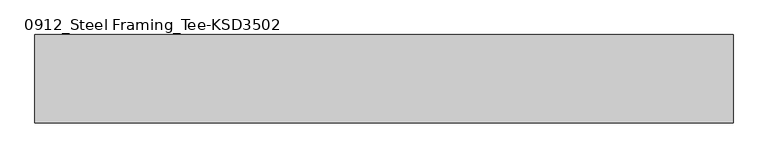
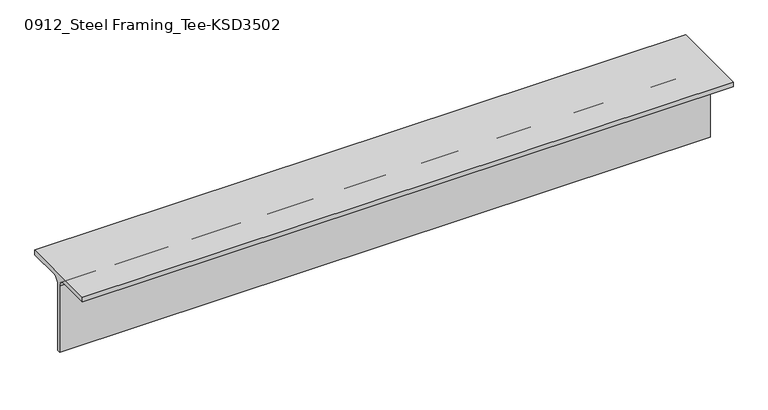
"""IFC4 building model written with IfcOpenShell, lengths in millimetres: member geometry, 0912_Steel Framing_Tee-KSD3502 : H_SB_ASB_CT-150x150x6.5x9."""

import ifcopenshell
import ifcopenshell.guid

model = None  # the IFC model being written
_history = None  # IfcOwnerHistory: only IFC2X3 demands one
_inside = {}  # id of a spatial element -> (the spatial element, [elements in it])
_under = {}  # id of a project, library or spatial element -> (it, [spatial elements below it])
_declared = {}  # id of a project -> (the project, [libraries it declares])
_typed = {}  # id of a type object -> (the type object, [elements of that type])
_made_of = {}  # id of a material, layer set ... -> (it, [elements and type objects made of it])


def new_model(schema):
    """Start an empty IFC model of exactly this schema.

    Asked for "IFC4X3", IfcOpenShell would pick the latest addendum, in which some entities
    have other attributes; the version numbers below select the first issue.
    IFC2X3 requires an IfcOwnerHistory on every rooted entity: one is made here for all.
    """
    global model, _history
    if schema == "IFC4X3":
        model = ifcopenshell.file(schema_version=(4, 3, 0, 0))
    else:
        model = ifcopenshell.file(schema=schema)
    _inside.clear()
    _under.clear()
    _declared.clear()
    _typed.clear()
    _made_of.clear()
    _history = None
    if model.schema == "IFC2X3":
        org = make("IfcOrganization", Name="unknown")
        user = make(
            "IfcPersonAndOrganization",
            ThePerson=make("IfcPerson", FamilyName="unknown"),
            TheOrganization=org,
        )
        app = make(
            "IfcApplication",
            ApplicationDeveloper=org,
            Version="unknown",
            ApplicationFullName="unknown",
            ApplicationIdentifier="unknown",
        )
        _history = make(
            "IfcOwnerHistory",
            OwningUser=user,
            OwningApplication=app,
            ChangeAction="ADDED",
            CreationDate=0,
        )
    return model


def make(cls, **values):
    """One entity of the class cls with the attributes given. An attribute that is None is left unset."""
    return model.create_entity(
        cls, **{name: value for name, value in values.items() if value is not None}
    )


def rooted(cls, **values):
    """An entity with a GlobalId (a new one), such as an element, a storey or a relation."""
    return make(cls, GlobalId=ifcopenshell.guid.new(), OwnerHistory=_history, **values)


def si_unit(unit_type, name, prefix=None):
    """IfcSIUnit, for example si_unit("LENGTHUNIT", "METRE", prefix="MILLI")."""
    return make("IfcSIUnit", UnitType=unit_type, Prefix=prefix, Name=name)


def assignment(units):
    """IfcUnitAssignment: the units of a project."""
    return None if units is None else make("IfcUnitAssignment", Units=units)


def point(xyz):
    """IfcCartesianPoint."""
    return None if xyz is None else make("IfcCartesianPoint", Coordinates=xyz)


def direction(xyz):
    """IfcDirection."""
    return None if xyz is None else make("IfcDirection", DirectionRatios=xyz)


def frame(location, z_axis=None, x_axis=None):
    """IfcAxis2Placement3D, a coordinate frame: its origin and axes. An axis left out is left unset."""
    return make(
        "IfcAxis2Placement3D",
        Location=point(location),
        Axis=direction(z_axis),
        RefDirection=direction(x_axis),
    )


def frame_2d(location, x_axis=None):
    """IfcAxis2Placement2D, a coordinate frame in the plane: its origin and x axis."""
    return make(
        "IfcAxis2Placement2D", Location=point(location), RefDirection=direction(x_axis)
    )


def origin():
    """The frame at (0, 0, 0) with its axes left unset."""
    return frame((0.0, 0.0, 0.0))


def place(relative_to, where):
    """IfcLocalPlacement: puts the frame where relative to a parent placement (None: the world)."""
    return make(
        "IfcLocalPlacement", PlacementRelTo=relative_to, RelativePlacement=where
    )


def context(
    kind, dimensions, precision=None, world=None, true_north=None, identifier=None
):
    """IfcGeometricRepresentationContext, for example the 3D "Model" context."""
    return make(
        "IfcGeometricRepresentationContext",
        ContextIdentifier=identifier,
        ContextType=kind,
        CoordinateSpaceDimension=dimensions,
        Precision=precision,
        WorldCoordinateSystem=world,
        TrueNorth=true_north,
    )


def project(units=None, contexts=None):
    """IfcProject with its units and contexts."""
    return rooted(
        "IfcProject",
        Name="project",
        RepresentationContexts=contexts,
        UnitsInContext=assignment(units),
    )


def spatial(cls, under=None, at=None, **own):
    """A site, building, storey or space (cls), placed at a placement, below another one or the project."""
    s = rooted(cls, ObjectPlacement=at, **own)
    if under is not None:
        _under.setdefault(under.id(), (under, []))[1].append(s)
    return s


def polyline(points):
    """IfcPolyline through the points."""
    return make("IfcPolyline", Points=[point(p) for p in points])


def circle_curve(where, radius):
    """IfcCircle in the frame where."""
    return make("IfcCircle", Position=where, Radius=radius)


def trimmed(basis, trim1, trim2, sense, master):
    """IfcTrimmedCurve: the piece of a basis curve between two trims."""
    return make(
        "IfcTrimmedCurve",
        BasisCurve=basis,
        Trim1=trim1,
        Trim2=trim2,
        SenseAgreement=sense,
        MasterRepresentation=master,
    )


def segment(curve, same_sense, transition):
    """IfcCompositeCurveSegment."""
    return make(
        "IfcCompositeCurveSegment",
        Transition=transition,
        SameSense=same_sense,
        ParentCurve=curve,
    )


def composite_curve(segments, self_intersect=None):
    """IfcCompositeCurve: segments joined end to end."""
    return make("IfcCompositeCurve", Segments=segments, SelfIntersect=self_intersect)


def outline(outer, holes=None, kind="AREA"):
    """IfcArbitraryClosedProfileDef: a profile drawn as a closed curve; with holes, ...WithVoids."""
    if holes is None:
        return make("IfcArbitraryClosedProfileDef", ProfileType=kind, OuterCurve=outer)
    return make(
        "IfcArbitraryProfileDefWithVoids",
        ProfileType=kind,
        OuterCurve=outer,
        InnerCurves=holes,
    )


def extrude(swept, where, along, depth):
    """IfcExtrudedAreaSolid: the profile swept, set in the frame where, extruded along a direction by depth."""
    return make(
        "IfcExtrudedAreaSolid",
        SweptArea=swept,
        Position=where,
        ExtrudedDirection=direction(along),
        Depth=depth,
    )


def shape(context_of_items, identifier, shape_type, items):
    """IfcShapeRepresentation: the items that make up one representation, for example the "Body"."""
    return make(
        "IfcShapeRepresentation",
        ContextOfItems=context_of_items,
        RepresentationIdentifier=identifier,
        RepresentationType=shape_type,
        Items=items,
    )


def source(mapping_origin, context_of_items, identifier, shape_type, items):
    """IfcRepresentationMap: a shape defined once, which mapped items show again and again."""
    return make(
        "IfcRepresentationMap",
        MappingOrigin=mapping_origin,
        MappedRepresentation=shape(context_of_items, identifier, shape_type, items),
    )


def transform(
    local_origin,
    x_axis=None,
    y_axis=None,
    z_axis=None,
    scale=None,
    scale2=None,
    scale3=None,
    uniform=True,
):
    """IfcCartesianTransformationOperator3D, or its non-uniform kind. x_axis, y_axis, z_axis: its Axis1, 2, 3."""
    if uniform:
        return make(
            "IfcCartesianTransformationOperator3D",
            Axis1=direction(x_axis),
            Axis2=direction(y_axis),
            LocalOrigin=point(local_origin),
            Scale=scale,
            Axis3=direction(z_axis),
        )
    return make(
        "IfcCartesianTransformationOperator3DnonUniform",
        Axis1=direction(x_axis),
        Axis2=direction(y_axis),
        LocalOrigin=point(local_origin),
        Scale=scale,
        Axis3=direction(z_axis),
        Scale2=scale2,
        Scale3=scale3,
    )


def mapped(mapping_source, mapping_target):
    """IfcMappedItem: shows the shape of a source again, moved by a transform."""
    return make(
        "IfcMappedItem", MappingSource=mapping_source, MappingTarget=mapping_target
    )


def made_of(thing, what):
    """Note that an element or type object is made of a material, layer set ...; save() writes the relation."""
    if what is not None:
        _made_of.setdefault(what.id(), (what, []))[1].append(thing)
    return thing


def element(
    cls,
    number,
    at=None,
    inside=None,
    cuts=None,
    type_object=None,
    material=None,
    context=None,
    identifier="Body",
    shape_type=None,
    held_by="IfcProductDefinitionShape",
    body=None,
    shapes=None,
    **own,
):
    """One element of the class cls, such as IfcWall. Its Tag is "e" and its number.

    at: its placement. inside: the storey or other place that contains it. cuts: it is an
    opening in that element (IfcRelVoidsElement). A single representation is given by context,
    identifier, shape_type and body (its items); several are given by shapes. held_by: the class
    of the entity that holds the representations. save() writes the other relations.
    """
    e = rooted(cls, Tag="e%d" % number, ObjectPlacement=at, **own)
    if body is not None:
        shapes = [shape(context, identifier, shape_type, body)]
    if shapes is not None:
        e.Representation = make(held_by, Representations=shapes)
    if inside is not None:
        _inside.setdefault(inside.id(), (inside, []))[1].append(e)
    if cuts is not None:
        rooted(
            "IfcRelVoidsElement", RelatingBuildingElement=cuts, RelatedOpeningElement=e
        )
    if type_object is not None:
        _typed.setdefault(type_object.id(), (type_object, []))[1].append(e)
    return made_of(e, material)


def aggregate(whole, parts):
    """IfcRelAggregates: a whole, such as a stair, and the parts it consists of."""
    return rooted("IfcRelAggregates", RelatingObject=whole, RelatedObjects=parts)


def save(model, path):
    """Write the relations noted so far, then the file.

    IfcRelAggregates (storeys below a building ...), IfcRelContainedInSpatialStructure (elements
    in a storey), IfcRelDefinesByType, IfcRelAssociatesMaterial and IfcRelDeclares: one each for
    every whole, place, type object, material and project.
    """
    for whole, parts in _under.values():
        aggregate(whole, parts)
    for where, things in _inside.values():
        rooted(
            "IfcRelContainedInSpatialStructure",
            RelatedElements=things,
            RelatingStructure=where,
        )
    for kind, things in _typed.values():
        rooted("IfcRelDefinesByType", RelatedObjects=things, RelatingType=kind)
    for what, things in _made_of.values():
        rooted("IfcRelAssociatesMaterial", RelatedObjects=things, RelatingMaterial=what)
    for by, libraries in _declared.values():
        rooted("IfcRelDeclares", RelatingContext=by, RelatedDefinitions=libraries)
    model.write(path)


def member_0912_steel_framing_tee_ksd3502_9b959b21(model_context):
    return source(origin(), model_context, "Body", "SweptSolid", [
        extrude(outline(composite_curve([segment(polyline([(-75.0, 75.0), (75.0, 75.0), (75.0, 66.0), (16.25, 66.0)]), True, "CONTINUOUS"), segment(trimmed(circle_curve(frame_2d((16.25, 53.0)), 13.0), [point((16.25, 66.0))], [point((3.25, 53.0))], True, "CARTESIAN"), True, "CONTINUOUS"), segment(polyline([(3.25, 53.0), (3.25, -75.0), (-3.25, -75.0), (-3.25, 53.0)]), True, "CONTINUOUS"), segment(trimmed(circle_curve(frame_2d((-16.25, 53.0)), 13.0), [point((-3.25, 53.0))], [point((-16.25, 66.0))], True, "CARTESIAN"), True, "CONTINUOUS"), segment(polyline([(-16.25, 66.0), (-75.0, 66.0), (-75.0, 75.0)]), True, "CONTINUOUS")], self_intersect=False)), frame((-701.75, 0.0, 0.0), z_axis=(1.0, 0.0, 0.0), x_axis=(0.0, 1.0, 0.0)), (0.0, 0.0, 1.0), 1186.2),
    ])


if __name__ == "__main__":
    model = new_model("IFC4")
    model_context = context("Model", 3, world=origin())
    ifc_project = project(units=[si_unit("LENGTHUNIT", "METRE", prefix="MILLI")], contexts=[model_context])
    site = spatial("IfcSite", under=ifc_project)
    building = spatial("IfcBuilding", under=site)
    placement = place(None, origin())
    member_0912_steel_framing_tee_ksd3502_shape = member_0912_steel_framing_tee_ksd3502_9b959b21(model_context)
    element("IfcMember", 1, ObjectType="0912_Steel Framing_Tee-KSD3502 : H_SB_ASB_CT-150x150x6.5x9", at=placement, inside=building, context=model_context, shape_type="MappedRepresentation", body=[
        mapped(member_0912_steel_framing_tee_ksd3502_shape, transform((0.0, 0.0, 0.0), x_axis=(1.0, 0.0, 0.0), y_axis=(0.0, 1.0, 0.0), z_axis=(0.0, 0.0, 1.0))),
    ])
    save(model, "model.ifc")

# Revit data of these elements
# Type "0912_Steel Framing_Tee-KSD3502 : H_SB_ASB_CT-150x150x6.5x9"
#   H_WM Code_1 = "S01AA003-00001 | Main Steel Structure Fabrication Work | Shelter/Building | Light Steel - Standard (30KG/M>Weight) | Material: (   )"
#   H_WM Code_2 = "S03AA029-00001 | Main Steel Structure Erection Work | Shelter/Building | Light Steel (30KG/M>Weight) | Material: (   )"
#   H_WM Code_3 = "S01AA010-00001 | Main Steel Structure Fabrication Work | Shelter/Building | Steel Painting/Coating | for Non-Fireproofed Steel Surface, Surface Preparation, Primer, Second & Final Coat | Material: (   )"
#   H_Q'ty Cal Type Tag = "SB-Q2"
#   Width = 15.0 cm
#   Web Thickness = 0.65 cm
#   Web Fillet = 1.3 cm
#   Section Area = 23.39 cm²
#   Perimeter = 0.60 m²/m
#   Nominal Weight = 18.40 kgf/m
#   Height = 15.0 cm
#   Flange Thickness = 0.9 cm
#   Centroid Vertical = 7.5 cm
#   Centroid Horizontal = 7.5 cm
#   Length [instance default] = 1.5000 m
#   Structural Material [instance default] = Steel, 45-345
#   Warping Constant = (empty or 0)
#   Torsional Moment of Inertia = 0
#   Section Name Key = ""
#   Plastic Modulus weak axis = 0
#   Plastic Modulus strong axis = 0
#   Moment of Inertia weak axis = 0
#   Moment of Inertia strong axis = 0
#   Elastic Modulus weak axis = 0
#   Elastic Modulus strong axis = 0
#   Bolt Spacing = 0
#   Assembly Code = ""
# Element 1 (IfcMember, "0912_Steel Framing_Tee-KSD3502 : H_SB_ASB_CT-150x150x6.5x9")
#   Structural Material = none
# Materials
#   "Steel, 45-345": class "Metal", colour RGB 189 187 185, transparency 0, Description = "Steel 345 MPa", Cost = 0
